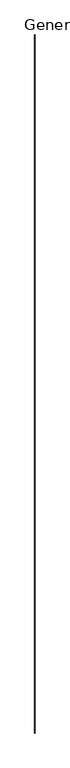
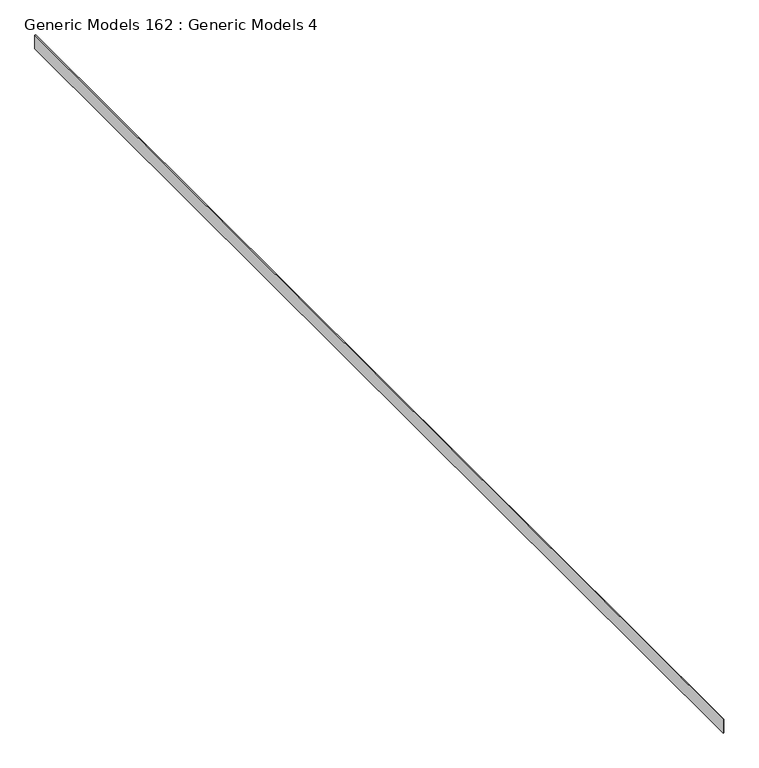
"""IFC4 building model written with IfcOpenShell, lengths in millimetres: proxy geometry, Generic Models 162 : Generic Models 4."""

import ifcopenshell
import ifcopenshell.guid

model = None  # the IFC model being written
_history = None  # IfcOwnerHistory: only IFC2X3 demands one
_inside = {}  # id of a spatial element -> (the spatial element, [elements in it])
_under = {}  # id of a project, library or spatial element -> (it, [spatial elements below it])
_declared = {}  # id of a project -> (the project, [libraries it declares])
_typed = {}  # id of a type object -> (the type object, [elements of that type])
_made_of = {}  # id of a material, layer set ... -> (it, [elements and type objects made of it])


def new_model(schema):
    """Start an empty IFC model of exactly this schema.

    Asked for "IFC4X3", IfcOpenShell would pick the latest addendum, in which some entities
    have other attributes; the version numbers below select the first issue.
    IFC2X3 requires an IfcOwnerHistory on every rooted entity: one is made here for all.
    """
    global model, _history
    if schema == "IFC4X3":
        model = ifcopenshell.file(schema_version=(4, 3, 0, 0))
    else:
        model = ifcopenshell.file(schema=schema)
    _inside.clear()
    _under.clear()
    _declared.clear()
    _typed.clear()
    _made_of.clear()
    _history = None
    if model.schema == "IFC2X3":
        org = make("IfcOrganization", Name="unknown")
        user = make(
            "IfcPersonAndOrganization",
            ThePerson=make("IfcPerson", FamilyName="unknown"),
            TheOrganization=org,
        )
        app = make(
            "IfcApplication",
            ApplicationDeveloper=org,
            Version="unknown",
            ApplicationFullName="unknown",
            ApplicationIdentifier="unknown",
        )
        _history = make(
            "IfcOwnerHistory",
            OwningUser=user,
            OwningApplication=app,
            ChangeAction="ADDED",
            CreationDate=0,
        )
    return model


def make(cls, **values):
    """One entity of the class cls with the attributes given. An attribute that is None is left unset."""
    return model.create_entity(
        cls, **{name: value for name, value in values.items() if value is not None}
    )


def rooted(cls, **values):
    """An entity with a GlobalId (a new one), such as an element, a storey or a relation."""
    return make(cls, GlobalId=ifcopenshell.guid.new(), OwnerHistory=_history, **values)


def si_unit(unit_type, name, prefix=None):
    """IfcSIUnit, for example si_unit("LENGTHUNIT", "METRE", prefix="MILLI")."""
    return make("IfcSIUnit", UnitType=unit_type, Prefix=prefix, Name=name)


def assignment(units):
    """IfcUnitAssignment: the units of a project."""
    return None if units is None else make("IfcUnitAssignment", Units=units)


def point(xyz):
    """IfcCartesianPoint."""
    return None if xyz is None else make("IfcCartesianPoint", Coordinates=xyz)


def direction(xyz):
    """IfcDirection."""
    return None if xyz is None else make("IfcDirection", DirectionRatios=xyz)


def frame(location, z_axis=None, x_axis=None):
    """IfcAxis2Placement3D, a coordinate frame: its origin and axes. An axis left out is left unset."""
    return make(
        "IfcAxis2Placement3D",
        Location=point(location),
        Axis=direction(z_axis),
        RefDirection=direction(x_axis),
    )


def origin():
    """The frame at (0, 0, 0) with its axes left unset."""
    return frame((0.0, 0.0, 0.0))


def place(relative_to, where):
    """IfcLocalPlacement: puts the frame where relative to a parent placement (None: the world)."""
    return make(
        "IfcLocalPlacement", PlacementRelTo=relative_to, RelativePlacement=where
    )


def context(
    kind, dimensions, precision=None, world=None, true_north=None, identifier=None
):
    """IfcGeometricRepresentationContext, for example the 3D "Model" context."""
    return make(
        "IfcGeometricRepresentationContext",
        ContextIdentifier=identifier,
        ContextType=kind,
        CoordinateSpaceDimension=dimensions,
        Precision=precision,
        WorldCoordinateSystem=world,
        TrueNorth=true_north,
    )


def project(units=None, contexts=None):
    """IfcProject with its units and contexts."""
    return rooted(
        "IfcProject",
        Name="project",
        RepresentationContexts=contexts,
        UnitsInContext=assignment(units),
    )


def spatial(cls, under=None, at=None, **own):
    """A site, building, storey or space (cls), placed at a placement, below another one or the project."""
    s = rooted(cls, ObjectPlacement=at, **own)
    if under is not None:
        _under.setdefault(under.id(), (under, []))[1].append(s)
    return s


def faces_of(points, faces, orient=None, outer=None):
    """IfcFace entities. A face is a list of loops; a loop is a list of indices into points, from 0.

    orient and outer hold one flag for each loop. By default every Orientation is true, the
    first loop of a face is its IfcFaceOuterBound and the others are IfcFaceBound.
    """
    made = []
    for i, loops in enumerate(faces):
        bounds = []
        for j, loop in enumerate(loops):
            is_outer = j == 0 if outer is None else outer[i][j]
            bounds.append(
                make(
                    "IfcFaceOuterBound" if is_outer else "IfcFaceBound",
                    Bound=make("IfcPolyLoop", Polygon=[points[k] for k in loop]),
                    Orientation=True if orient is None else orient[i][j],
                )
            )
        made.append(make("IfcFace", Bounds=bounds))
    return made


def faceted_brep(points, faces, orient=None, outer=None, voids=None):
    """IfcFacetedBrep: a solid bounded by flat faces; with voids (closed shells), ...WithVoids."""
    shared = [point(p) for p in points]
    hull = make("IfcClosedShell", CfsFaces=faces_of(shared, faces, orient, outer))
    if voids is None:
        return make("IfcFacetedBrep", Outer=hull)
    return make(
        "IfcFacetedBrepWithVoids",
        Outer=hull,
        Voids=[
            make(cls, CfsFaces=faces_of(shared, fs, o, b)) for cls, fs, o, b in voids
        ],
    )


def shape(context_of_items, identifier, shape_type, items):
    """IfcShapeRepresentation: the items that make up one representation, for example the "Body"."""
    return make(
        "IfcShapeRepresentation",
        ContextOfItems=context_of_items,
        RepresentationIdentifier=identifier,
        RepresentationType=shape_type,
        Items=items,
    )


def source(mapping_origin, context_of_items, identifier, shape_type, items):
    """IfcRepresentationMap: a shape defined once, which mapped items show again and again."""
    return make(
        "IfcRepresentationMap",
        MappingOrigin=mapping_origin,
        MappedRepresentation=shape(context_of_items, identifier, shape_type, items),
    )


def transform(
    local_origin,
    x_axis=None,
    y_axis=None,
    z_axis=None,
    scale=None,
    scale2=None,
    scale3=None,
    uniform=True,
):
    """IfcCartesianTransformationOperator3D, or its non-uniform kind. x_axis, y_axis, z_axis: its Axis1, 2, 3."""
    if uniform:
        return make(
            "IfcCartesianTransformationOperator3D",
            Axis1=direction(x_axis),
            Axis2=direction(y_axis),
            LocalOrigin=point(local_origin),
            Scale=scale,
            Axis3=direction(z_axis),
        )
    return make(
        "IfcCartesianTransformationOperator3DnonUniform",
        Axis1=direction(x_axis),
        Axis2=direction(y_axis),
        LocalOrigin=point(local_origin),
        Scale=scale,
        Axis3=direction(z_axis),
        Scale2=scale2,
        Scale3=scale3,
    )


def mapped(mapping_source, mapping_target):
    """IfcMappedItem: shows the shape of a source again, moved by a transform."""
    return make(
        "IfcMappedItem", MappingSource=mapping_source, MappingTarget=mapping_target
    )


def made_of(thing, what):
    """Note that an element or type object is made of a material, layer set ...; save() writes the relation."""
    if what is not None:
        _made_of.setdefault(what.id(), (what, []))[1].append(thing)
    return thing


def element(
    cls,
    number,
    at=None,
    inside=None,
    cuts=None,
    type_object=None,
    material=None,
    context=None,
    identifier="Body",
    shape_type=None,
    held_by="IfcProductDefinitionShape",
    body=None,
    shapes=None,
    **own,
):
    """One element of the class cls, such as IfcWall. Its Tag is "e" and its number.

    at: its placement. inside: the storey or other place that contains it. cuts: it is an
    opening in that element (IfcRelVoidsElement). A single representation is given by context,
    identifier, shape_type and body (its items); several are given by shapes. held_by: the class
    of the entity that holds the representations. save() writes the other relations.
    """
    e = rooted(cls, Tag="e%d" % number, ObjectPlacement=at, **own)
    if body is not None:
        shapes = [shape(context, identifier, shape_type, body)]
    if shapes is not None:
        e.Representation = make(held_by, Representations=shapes)
    if inside is not None:
        _inside.setdefault(inside.id(), (inside, []))[1].append(e)
    if cuts is not None:
        rooted(
            "IfcRelVoidsElement", RelatingBuildingElement=cuts, RelatedOpeningElement=e
        )
    if type_object is not None:
        _typed.setdefault(type_object.id(), (type_object, []))[1].append(e)
    return made_of(e, material)


def aggregate(whole, parts):
    """IfcRelAggregates: a whole, such as a stair, and the parts it consists of."""
    return rooted("IfcRelAggregates", RelatingObject=whole, RelatedObjects=parts)


def save(model, path):
    """Write the relations noted so far, then the file.

    IfcRelAggregates (storeys below a building ...), IfcRelContainedInSpatialStructure (elements
    in a storey), IfcRelDefinesByType, IfcRelAssociatesMaterial and IfcRelDeclares: one each for
    every whole, place, type object, material and project.
    """
    for whole, parts in _under.values():
        aggregate(whole, parts)
    for where, things in _inside.values():
        rooted(
            "IfcRelContainedInSpatialStructure",
            RelatedElements=things,
            RelatingStructure=where,
        )
    for kind, things in _typed.values():
        rooted("IfcRelDefinesByType", RelatedObjects=things, RelatingType=kind)
    for what, things in _made_of.values():
        rooted("IfcRelAssociatesMaterial", RelatedObjects=things, RelatingMaterial=what)
    for by, libraries in _declared.values():
        rooted("IfcRelDeclares", RelatingContext=by, RelatedDefinitions=libraries)
    model.write(path)


def generic_models_162_generic_models_4_41cdbdbc(model_context):
    return source(origin(), model_context, "Body", "Brep", [
        faceted_brep([(-10237.6972239, -5493.3230338, 122946.1234874), (-10237.6972239, -5493.3230338, 122897.0249647), (-10237.6972239, -5493.3230338, 122842.82201), (-10237.6972239, -5493.3230338, 122820.8249647), (-10237.6972239, -5493.3230338, 122793.7234874), (-10236.1097239, -5493.3230338, 122793.7234874), (-10231.3472239, -5493.3230338, 122793.7234874), (-10231.3472239, -5493.3230338, 122946.1234874), (-10237.6972239, 7054.2769662, 122946.1234874), (-10231.3472239, 7054.2769662, 122946.1234874), (-10231.3472239, 7054.2769662, 122793.7234874), (-10236.1097239, 7054.2769662, 122793.7234874), (-10237.6972239, 7054.2769662, 122793.7234874), (-10237.6972239, 7054.2769662, 122820.8249648), (-10237.6972239, 7054.2769662, 122842.82201), (-10237.6972239, 7054.2769662, 122897.0249648)], [[[0, 1, 2, 3, 4, 5, 6, 7]], [[8, 9, 10, 11, 12, 13, 14, 15]], [[4, 3, 2, 1, 0, 8, 15, 14, 13, 12]], [[6, 5, 4, 12, 11, 10]], [[7, 6, 10, 9]], [[0, 7, 9, 8]]]),
    ])


if __name__ == "__main__":
    model = new_model("IFC4")
    model_context = context("Model", 3, world=origin())
    ifc_project = project(units=[si_unit("LENGTHUNIT", "METRE", prefix="MILLI")], contexts=[model_context])
    site = spatial("IfcSite", under=ifc_project)
    building = spatial("IfcBuilding", under=site)
    placement = place(None, origin())
    generic_models_162_generic_models_4_shape = generic_models_162_generic_models_4_41cdbdbc(model_context)
    element("IfcBuildingElementProxy", 1, Name="Generic Models 162 : Generic Models 4", ObjectType="Generic Models 162 : Generic Models 4", at=placement, inside=building, context=model_context, shape_type="MappedRepresentation", body=[
        mapped(generic_models_162_generic_models_4_shape, transform((0.0, 0.0, 0.0), x_axis=(1.0, 0.0, 0.0), y_axis=(0.0, 1.0, 0.0), z_axis=(0.0, 0.0, 1.0))),
    ])
    save(model, "model.ifc")

# Revit data of these elements
# Element 1 (IfcBuildingElementProxy, "Generic Models 162 : Generic Models 4")
#   Materials on its faces: "_STEEL BASE PLATE AT EACH RAILING POST (SEE STRUCT. DWGS)"
# Materials
#   "_STEEL BASE PLATE AT EACH RAILING POST (SEE STRUCT. DWGS)": class "Generic", colour RGB 233 233 233, transparency 0, Cost = 0
